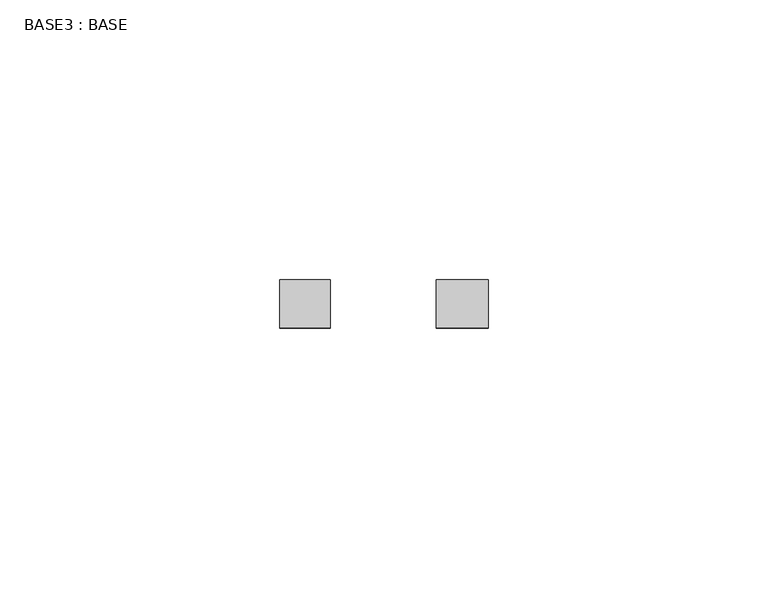
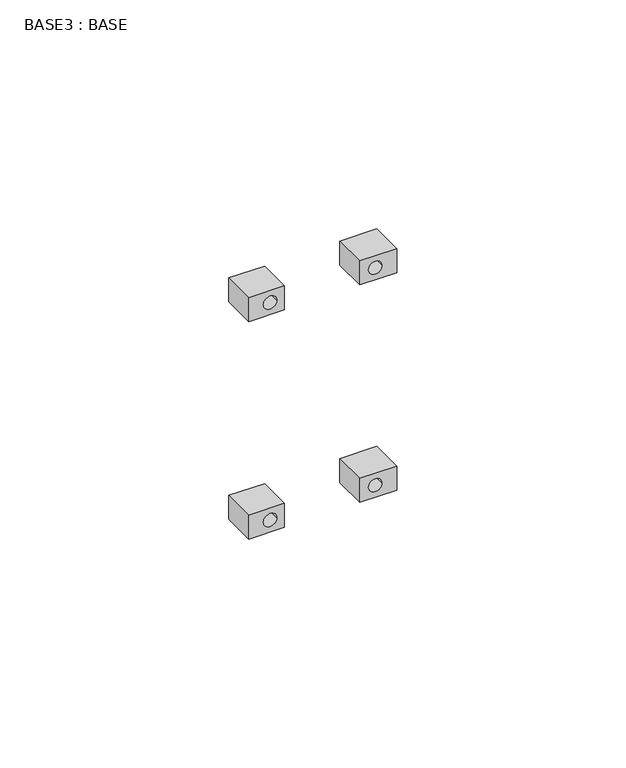
"""IFC4 building model written with IfcOpenShell, lengths in millimetres: proxy geometry, BASE3 : BASE."""

from ifc_helpers import new_model, si_unit, point, frame, frame_2d, origin, place, context, project, spatial, polyline, circle_curve, trimmed, segment, composite_curve, outline, extrude, source, transform, mapped, element, save


def base3_base_5e775e04(model_context):
    return source(origin(), model_context, "Body", "SweptSolid", [
        extrude(outline(polyline([(59.8, 2465.0719295), (59.8, 2474.3719295), (66.2, 2474.3719295), (66.2, 2465.0719295), (59.8, 2465.0719295)]), holes=[composite_curve([segment(trimmed(circle_curve(frame_2d((63.0, 2468.9719295)), 1.7), [point((63.0, 2467.2719295))], [point((63.0, 2470.6719295))], True, "CARTESIAN"), True, "CONTINUOUS"), segment(trimmed(circle_curve(frame_2d((63.0, 2468.9719295)), 1.7), [point((63.0, 2470.6719295))], [point((63.0, 2467.2719295))], True, "CARTESIAN"), True, "CONTINUOUS")], self_intersect=False)]), frame((0.0, 1296.9192449, 0.0), z_axis=(0.0, 1.0, 0.0), x_axis=(0.0, 0.0, 1.0)), (0.0, 0.0, 1.0), 8.6306009),
        extrude(outline(polyline([(59.8, 2437.0719295), (59.8, 2446.0719295), (66.2, 2446.0719295), (66.2, 2437.0719295), (59.8, 2437.0719295)]), holes=[composite_curve([segment(trimmed(circle_curve(frame_2d((63.0, 2442.4719295)), 1.7), [point((63.0, 2444.1719295))], [point((63.0, 2440.7719295))], True, "CARTESIAN"), True, "CONTINUOUS"), segment(trimmed(circle_curve(frame_2d((63.0, 2442.4719295)), 1.7), [point((63.0, 2440.7719295))], [point((63.0, 2444.1719295))], True, "CARTESIAN"), True, "CONTINUOUS")], self_intersect=False)]), frame((0.0, 1296.9192449, 0.0), z_axis=(0.0, 1.0, 0.0), x_axis=(0.0, 0.0, 1.0)), (0.0, 0.0, 1.0), 8.6306009),
        extrude(outline(polyline([(1.8, 2465.0719295), (1.8, 2474.3719295), (8.2, 2474.3719295), (8.2, 2465.0719295), (1.8, 2465.0719295)]), holes=[composite_curve([segment(trimmed(circle_curve(frame_2d((5.0, 2468.9719295)), 1.7), [point((5.0, 2470.6719295))], [point((5.0, 2467.2719295))], True, "CARTESIAN"), True, "CONTINUOUS"), segment(trimmed(circle_curve(frame_2d((5.0, 2468.9719295)), 1.7), [point((5.0, 2467.2719295))], [point((5.0, 2470.6719295))], True, "CARTESIAN"), True, "CONTINUOUS")], self_intersect=False)]), frame((0.0, 1296.9192449, 0.0), z_axis=(0.0, 1.0, 0.0), x_axis=(0.0, 0.0, 1.0)), (0.0, 0.0, 1.0), 8.6306009),
        extrude(outline(polyline([(1.8, 2446.0719295), (8.2, 2446.0719295), (8.2, 2437.0719295), (1.8, 2437.0719295), (1.8, 2446.0719295)]), holes=[composite_curve([segment(trimmed(circle_curve(frame_2d((5.0, 2442.4719295)), 1.7), [point((5.0, 2444.1719295))], [point((5.0, 2440.7719295))], True, "CARTESIAN"), True, "CONTINUOUS"), segment(trimmed(circle_curve(frame_2d((5.0, 2442.4719295)), 1.7), [point((5.0, 2440.7719295))], [point((5.0, 2444.1719295))], True, "CARTESIAN"), True, "CONTINUOUS")], self_intersect=False)]), frame((0.0, 1296.9192449, 0.0), z_axis=(0.0, 1.0, 0.0), x_axis=(0.0, 0.0, 1.0)), (0.0, 0.0, 1.0), 8.6306009),
    ])


if __name__ == "__main__":
    model = new_model("IFC4")
    model_context = context("Model", 3, world=origin())
    ifc_project = project(units=[si_unit("LENGTHUNIT", "METRE", prefix="MILLI")], contexts=[model_context])
    site = spatial("IfcSite", under=ifc_project)
    building = spatial("IfcBuilding", under=site)
    placement = place(None, origin())
    base3_base_shape = base3_base_5e775e04(model_context)
    element("IfcBuildingElementProxy", 1, Name="BASE3 : BASE", ObjectType="BASE3 : BASE", at=placement, inside=building, context=model_context, shape_type="MappedRepresentation", body=[
        mapped(base3_base_shape, transform((0.0, 0.0, 0.0), x_axis=(1.0, 0.0, 0.0), y_axis=(0.0, 1.0, 0.0), z_axis=(0.0, 0.0, 1.0))),
    ])
    save(model, "model.ifc")

# Revit data of these elements
# Element 1 (IfcBuildingElementProxy, "BASE3 : BASE")
#   Materials on its faces: ".BOX FUNDO"
# Materials
#   ".BOX FUNDO": class "Vidro", colour RGB 236 240 239, transparency 0.15, Cost = 0
